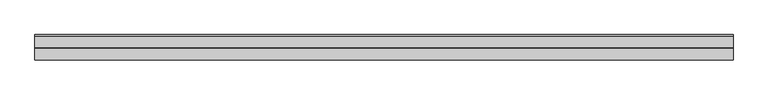
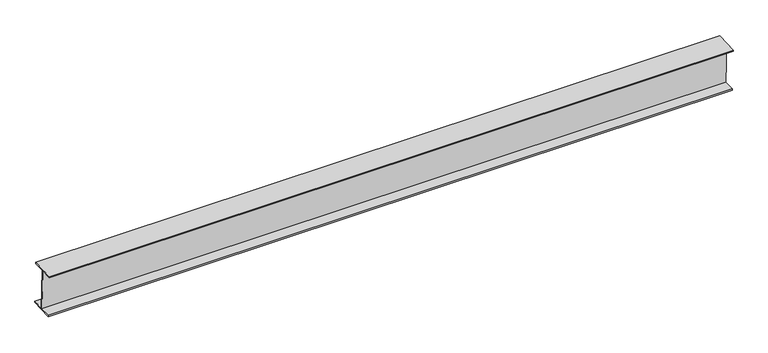
"""IFC4 building model written with IfcOpenShell, lengths in millimetres: proxy geometry, Generic Models 7:Generic Models 1:8:Generic Models 1:8 : Generic Models 7:Generic Models 1:337419:4 : Generic Models 7:Generic Models 1:8:Generic Models 1:8 : Generic Models 7:Generic Models 1:337419:315935."""

from ifc_helpers import new_model, si_unit, frame, origin, place, context, project, spatial, polyline, outline, extrude, source, transform, mapped, element, save


def generic_models_b0282a17(model_context):
    return source(origin(), model_context, "Body", "SweptSolid", [
        extrude(outline(polyline([(-578771.5288802, 3670.9066459), (-578771.8989757, 3679.7889389), (-578607.1996709, 3686.65141), (-578606.8295754, 3677.7691169), (-578686.0703802, 3674.4674167), (-578673.910098, 3382.6206461), (-578594.6692934, 3385.9223463), (-578594.2991979, 3377.0400533), (-578758.9985027, 3370.1775822), (-578759.3685982, 3379.0598752), (-578679.8739233, 3382.3721534), (-578692.0342055, 3674.218924), (-578771.5288802, 3670.9066459)])), frame((591306.0367239, 0.0, 0.0), z_axis=(1.0, 0.0, 0.0), x_axis=(0.0, 1.0, 0.0)), (0.0, 0.0, 1.0), 4876.8),
    ])


if __name__ == "__main__":
    model = new_model("IFC4")
    model_context = context("Model", 3, world=origin())
    ifc_project = project(units=[si_unit("LENGTHUNIT", "METRE", prefix="MILLI")], contexts=[model_context])
    site = spatial("IfcSite", under=ifc_project)
    building = spatial("IfcBuilding", under=site)
    placement = place(None, origin())
    generic_models_shape = generic_models_b0282a17(model_context)
    element("IfcBuildingElementProxy", 1, Name="Generic Models 7:Generic Models 1:8:Generic Models 1:8 : Generic Models 7:Generic Models 1:337419:4 : Generic Models 7:Generic Models 1:8:Generic Models 1:8 : Generic Models 7:Generic Models 1:337419:315935", ObjectType="Generic Models 7:Generic Models 1:8:Generic Models 1:8 : Generic Models 7:Generic Models 1:337419:4 : Generic Models 7:Generic Models 1:8:Generic Models 1:8 : Generic Models 7:Generic Models 1:337419:315935", at=placement, inside=building, context=model_context, shape_type="MappedRepresentation", body=[
        mapped(generic_models_shape, transform((0.0, 0.0, 0.0), x_axis=(1.0, 0.0, 0.0), y_axis=(0.0, 1.0, 0.0), z_axis=(0.0, 0.0, 1.0))),
    ])
    save(model, "model.ifc")

# Revit data of these elements
# Type "Generic Models 7:Generic Models 1:8:Generic Models 1:8 : Generic Models 7:Generic Models 1:337419:4 : Generic Models 7:Generic Models 1:8:Generic Models 1:8 : Generic Models 7:Generic Models 1:337419:315935"
#   NameOverride = "Generic Models 7:Generic Models 1:8:Generic Models 1:8 : Generic Models 7:Generic Models 1:337419:315935"
#   ObjectTypeOverride = "Generic Models 1:8 : Generic Models 7:Generic Models 1:337419"
#   Reference = "Generic Models 1"
#   Tag = "315935"
# Element 1 (IfcBuildingElementProxy, "Generic Models 7:Generic Models 1:8:Generic Models 1:8 : Generic Models 7:Generic Models 1:337419:4 : Generic Models 7:Generic Models 1:8:Generic Models 1:8 : Generic Models 7:Generic Models 1:337419:315935")
#   Materials on its faces: "STRUCTURAL STEEL - SEE STRUCT. DWGS"
# Materials
#   "STRUCTURAL STEEL - SEE STRUCT. DWGS": class "Metal", colour RGB 189 187 185, transparency 0, Description = "Structural steel 50ksi", Cost = 0
